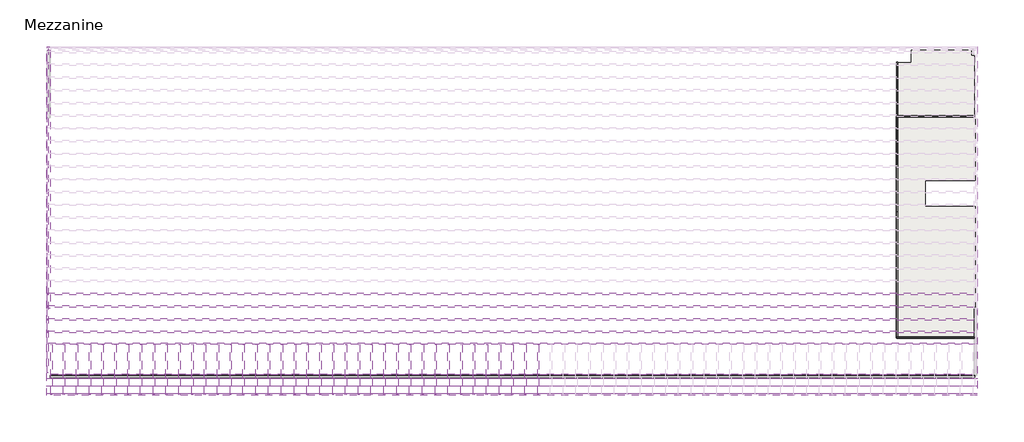
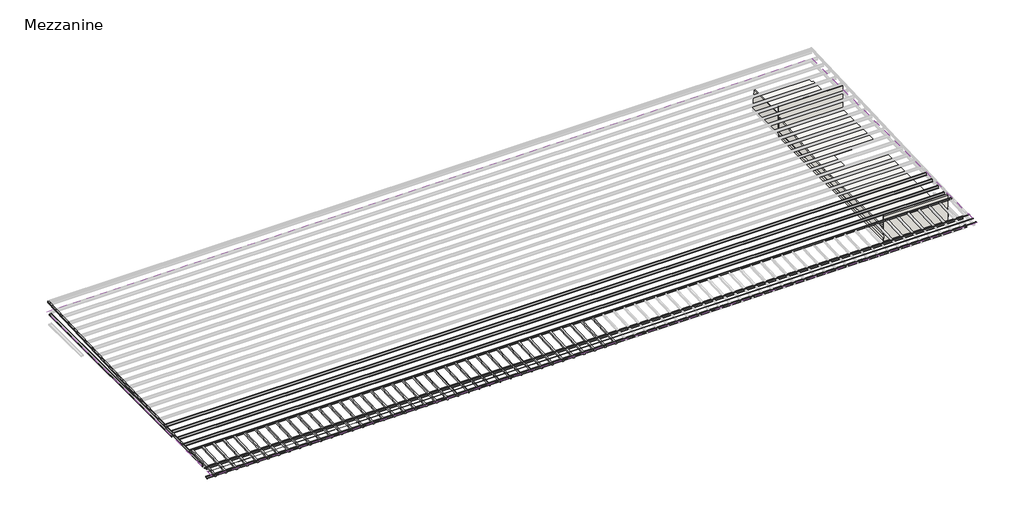
# One storey, part 1 of 2: 51 beams, 4 walls, 2 slabs, 1 roof.
"""IFC4 building model written with IfcOpenShell, lengths in millimetres."""

import ifcopenshell
import ifcopenshell.guid

model = None  # the IFC model being written
_history = None  # IfcOwnerHistory: only IFC2X3 demands one
_inside = {}  # id of a spatial element -> (the spatial element, [elements in it])
_under = {}  # id of a project, library or spatial element -> (it, [spatial elements below it])
_declared = {}  # id of a project -> (the project, [libraries it declares])
_typed = {}  # id of a type object -> (the type object, [elements of that type])
_made_of = {}  # id of a material, layer set ... -> (it, [elements and type objects made of it])


def new_model(schema):
    """Start an empty IFC model of exactly this schema.

    Asked for "IFC4X3", IfcOpenShell would pick the latest addendum, in which some entities
    have other attributes; the version numbers below select the first issue.
    IFC2X3 requires an IfcOwnerHistory on every rooted entity: one is made here for all.
    """
    global model, _history
    if schema == "IFC4X3":
        model = ifcopenshell.file(schema_version=(4, 3, 0, 0))
    else:
        model = ifcopenshell.file(schema=schema)
    _inside.clear()
    _under.clear()
    _declared.clear()
    _typed.clear()
    _made_of.clear()
    _history = None
    if model.schema == "IFC2X3":
        org = make("IfcOrganization", Name="unknown")
        user = make(
            "IfcPersonAndOrganization",
            ThePerson=make("IfcPerson", FamilyName="unknown"),
            TheOrganization=org,
        )
        app = make(
            "IfcApplication",
            ApplicationDeveloper=org,
            Version="unknown",
            ApplicationFullName="unknown",
            ApplicationIdentifier="unknown",
        )
        _history = make(
            "IfcOwnerHistory",
            OwningUser=user,
            OwningApplication=app,
            ChangeAction="ADDED",
            CreationDate=0,
        )
    return model


def make(cls, **values):
    """One entity of the class cls with the attributes given. An attribute that is None is left unset."""
    return model.create_entity(
        cls, **{name: value for name, value in values.items() if value is not None}
    )


def rooted(cls, **values):
    """An entity with a GlobalId (a new one), such as an element, a storey or a relation."""
    return make(cls, GlobalId=ifcopenshell.guid.new(), OwnerHistory=_history, **values)


def si_unit(unit_type, name, prefix=None):
    """IfcSIUnit, for example si_unit("LENGTHUNIT", "METRE", prefix="MILLI")."""
    return make("IfcSIUnit", UnitType=unit_type, Prefix=prefix, Name=name)


def assignment(units):
    """IfcUnitAssignment: the units of a project."""
    return None if units is None else make("IfcUnitAssignment", Units=units)


def point(xyz):
    """IfcCartesianPoint."""
    return None if xyz is None else make("IfcCartesianPoint", Coordinates=xyz)


def direction(xyz):
    """IfcDirection."""
    return None if xyz is None else make("IfcDirection", DirectionRatios=xyz)


def frame(location, z_axis=None, x_axis=None):
    """IfcAxis2Placement3D, a coordinate frame: its origin and axes. An axis left out is left unset."""
    return make(
        "IfcAxis2Placement3D",
        Location=point(location),
        Axis=direction(z_axis),
        RefDirection=direction(x_axis),
    )


def frame_2d(location, x_axis=None):
    """IfcAxis2Placement2D, a coordinate frame in the plane: its origin and x axis."""
    return make(
        "IfcAxis2Placement2D", Location=point(location), RefDirection=direction(x_axis)
    )


def origin():
    """The frame at (0, 0, 0) with its axes left unset."""
    return frame((0.0, 0.0, 0.0))


def place(relative_to, where):
    """IfcLocalPlacement: puts the frame where relative to a parent placement (None: the world)."""
    return make(
        "IfcLocalPlacement", PlacementRelTo=relative_to, RelativePlacement=where
    )


def context(
    kind, dimensions, precision=None, world=None, true_north=None, identifier=None
):
    """IfcGeometricRepresentationContext, for example the 3D "Model" context."""
    return make(
        "IfcGeometricRepresentationContext",
        ContextIdentifier=identifier,
        ContextType=kind,
        CoordinateSpaceDimension=dimensions,
        Precision=precision,
        WorldCoordinateSystem=world,
        TrueNorth=true_north,
    )


def project(units=None, contexts=None):
    """IfcProject with its units and contexts."""
    return rooted(
        "IfcProject",
        Name="project",
        RepresentationContexts=contexts,
        UnitsInContext=assignment(units),
    )


def spatial(cls, under=None, at=None, **own):
    """A site, building, storey or space (cls), placed at a placement, below another one or the project."""
    s = rooted(cls, ObjectPlacement=at, **own)
    if under is not None:
        _under.setdefault(under.id(), (under, []))[1].append(s)
    return s


def polyline(points):
    """IfcPolyline through the points."""
    return make("IfcPolyline", Points=[point(p) for p in points])


def circle_curve(where, radius):
    """IfcCircle in the frame where."""
    return make("IfcCircle", Position=where, Radius=radius)


def trimmed(basis, trim1, trim2, sense, master):
    """IfcTrimmedCurve: the piece of a basis curve between two trims."""
    return make(
        "IfcTrimmedCurve",
        BasisCurve=basis,
        Trim1=trim1,
        Trim2=trim2,
        SenseAgreement=sense,
        MasterRepresentation=master,
    )


def segment(curve, same_sense, transition):
    """IfcCompositeCurveSegment."""
    return make(
        "IfcCompositeCurveSegment",
        Transition=transition,
        SameSense=same_sense,
        ParentCurve=curve,
    )


def composite_curve(segments, self_intersect=None):
    """IfcCompositeCurve: segments joined end to end."""
    return make("IfcCompositeCurve", Segments=segments, SelfIntersect=self_intersect)


def outline(outer, holes=None, kind="AREA"):
    """IfcArbitraryClosedProfileDef: a profile drawn as a closed curve; with holes, ...WithVoids."""
    if holes is None:
        return make("IfcArbitraryClosedProfileDef", ProfileType=kind, OuterCurve=outer)
    return make(
        "IfcArbitraryProfileDefWithVoids",
        ProfileType=kind,
        OuterCurve=outer,
        InnerCurves=holes,
    )


def extrude(swept, where, along, depth):
    """IfcExtrudedAreaSolid: the profile swept, set in the frame where, extruded along a direction by depth."""
    return make(
        "IfcExtrudedAreaSolid",
        SweptArea=swept,
        Position=where,
        ExtrudedDirection=direction(along),
        Depth=depth,
    )


def faces_of(points, faces, orient=None, outer=None):
    """IfcFace entities. A face is a list of loops; a loop is a list of indices into points, from 0.

    orient and outer hold one flag for each loop. By default every Orientation is true, the
    first loop of a face is its IfcFaceOuterBound and the others are IfcFaceBound.
    """
    made = []
    for i, loops in enumerate(faces):
        bounds = []
        for j, loop in enumerate(loops):
            is_outer = j == 0 if outer is None else outer[i][j]
            bounds.append(
                make(
                    "IfcFaceOuterBound" if is_outer else "IfcFaceBound",
                    Bound=make("IfcPolyLoop", Polygon=[points[k] for k in loop]),
                    Orientation=True if orient is None else orient[i][j],
                )
            )
        made.append(make("IfcFace", Bounds=bounds))
    return made


def faceted_brep(points, faces, orient=None, outer=None, voids=None):
    """IfcFacetedBrep: a solid bounded by flat faces; with voids (closed shells), ...WithVoids."""
    shared = [point(p) for p in points]
    hull = make("IfcClosedShell", CfsFaces=faces_of(shared, faces, orient, outer))
    if voids is None:
        return make("IfcFacetedBrep", Outer=hull)
    return make(
        "IfcFacetedBrepWithVoids",
        Outer=hull,
        Voids=[
            make(cls, CfsFaces=faces_of(shared, fs, o, b)) for cls, fs, o, b in voids
        ],
    )


def shape(context_of_items, identifier, shape_type, items):
    """IfcShapeRepresentation: the items that make up one representation, for example the "Body"."""
    return make(
        "IfcShapeRepresentation",
        ContextOfItems=context_of_items,
        RepresentationIdentifier=identifier,
        RepresentationType=shape_type,
        Items=items,
    )


def source(mapping_origin, context_of_items, identifier, shape_type, items):
    """IfcRepresentationMap: a shape defined once, which mapped items show again and again."""
    return make(
        "IfcRepresentationMap",
        MappingOrigin=mapping_origin,
        MappedRepresentation=shape(context_of_items, identifier, shape_type, items),
    )


def transform(
    local_origin,
    x_axis=None,
    y_axis=None,
    z_axis=None,
    scale=None,
    scale2=None,
    scale3=None,
    uniform=True,
):
    """IfcCartesianTransformationOperator3D, or its non-uniform kind. x_axis, y_axis, z_axis: its Axis1, 2, 3."""
    if uniform:
        return make(
            "IfcCartesianTransformationOperator3D",
            Axis1=direction(x_axis),
            Axis2=direction(y_axis),
            LocalOrigin=point(local_origin),
            Scale=scale,
            Axis3=direction(z_axis),
        )
    return make(
        "IfcCartesianTransformationOperator3DnonUniform",
        Axis1=direction(x_axis),
        Axis2=direction(y_axis),
        LocalOrigin=point(local_origin),
        Scale=scale,
        Axis3=direction(z_axis),
        Scale2=scale2,
        Scale3=scale3,
    )


def mapped(mapping_source, mapping_target):
    """IfcMappedItem: shows the shape of a source again, moved by a transform."""
    return make(
        "IfcMappedItem", MappingSource=mapping_source, MappingTarget=mapping_target
    )


def made_of(thing, what):
    """Note that an element or type object is made of a material, layer set ...; save() writes the relation."""
    if what is not None:
        _made_of.setdefault(what.id(), (what, []))[1].append(thing)
    return thing


def element(
    cls,
    number,
    at=None,
    inside=None,
    cuts=None,
    type_object=None,
    material=None,
    context=None,
    identifier="Body",
    shape_type=None,
    held_by="IfcProductDefinitionShape",
    body=None,
    shapes=None,
    **own,
):
    """One element of the class cls, such as IfcWall. Its Tag is "e" and its number.

    at: its placement. inside: the storey or other place that contains it. cuts: it is an
    opening in that element (IfcRelVoidsElement). A single representation is given by context,
    identifier, shape_type and body (its items); several are given by shapes. held_by: the class
    of the entity that holds the representations. save() writes the other relations.
    """
    e = rooted(cls, Tag="e%d" % number, ObjectPlacement=at, **own)
    if body is not None:
        shapes = [shape(context, identifier, shape_type, body)]
    if shapes is not None:
        e.Representation = make(held_by, Representations=shapes)
    if inside is not None:
        _inside.setdefault(inside.id(), (inside, []))[1].append(e)
    if cuts is not None:
        rooted(
            "IfcRelVoidsElement", RelatingBuildingElement=cuts, RelatedOpeningElement=e
        )
    if type_object is not None:
        _typed.setdefault(type_object.id(), (type_object, []))[1].append(e)
    return made_of(e, material)


def aggregate(whole, parts):
    """IfcRelAggregates: a whole, such as a stair, and the parts it consists of."""
    return rooted("IfcRelAggregates", RelatingObject=whole, RelatedObjects=parts)


def save(model, path):
    """Write the relations noted so far, then the file.

    IfcRelAggregates (storeys below a building ...), IfcRelContainedInSpatialStructure (elements
    in a storey), IfcRelDefinesByType, IfcRelAssociatesMaterial and IfcRelDeclares: one each for
    every whole, place, type object, material and project.
    """
    for whole, parts in _under.values():
        aggregate(whole, parts)
    for where, things in _inside.values():
        rooted(
            "IfcRelContainedInSpatialStructure",
            RelatedElements=things,
            RelatingStructure=where,
        )
    for kind, things in _typed.values():
        rooted("IfcRelDefinesByType", RelatedObjects=things, RelatingType=kind)
    for what, things in _made_of.values():
        rooted("IfcRelAssociatesMaterial", RelatedObjects=things, RelatingMaterial=what)
    for by, libraries in _declared.values():
        rooted("IfcRelDeclares", RelatingContext=by, RelatedDefinitions=libraries)
    model.write(path)


def dimension_lumber_5_5_x_7_5_glulam_5a1f9f63(model_context):
    return source(origin(), model_context, "Body", "SweptSolid", [
        extrude(outline(polyline([(2439.95575, 69.85), (2439.95575, -69.85), (-2389.02875, -69.85), (-2389.02875, 69.85), (2439.95575, 69.85)])), frame((0.0, 0.0, -95.25), z_axis=(0.0, 0.0, 1.0), x_axis=(1.0, 0.0, 0.0)), (0.0, 0.0, 1.0), 190.5),
    ])


def beam_b6572ddd(model_context):
    return source(origin(), model_context, "Body", "SweptSolid", [
        extrude(outline(composite_curve([segment(polyline([(87.5109375, 101.6), (99.7560415, 87.0068534), (97.6278742, 85.221109), (86.2154765, 98.821875), (3.3005807, 98.821875)]), True, "CONTINUOUS"), segment(trimmed(circle_curve(frame_2d((3.3741066, 96.8381931)), 1.9850441), [point((3.3005807, 98.821875))], [point((1.3890625, 96.8381931))], True, "CARTESIAN"), True, "CONTINUOUS"), segment(polyline([(1.3890625, 96.8381931), (1.3890625, -96.8389339)]), True, "CONTINUOUS"), segment(trimmed(circle_curve(frame_2d((3.3748024, -96.8389339)), 1.9857399), [point((1.3890625, -96.8389339))], [point((3.2694106, -98.821875))], True, "CARTESIAN"), True, "CONTINUOUS"), segment(polyline([(3.2694106, -98.821875), (86.2154765, -98.821875), (97.6510975, -85.1934327), (99.7792647, -86.979177), (87.5109375, -101.6), (3.3734375, -101.6)]), True, "CONTINUOUS"), segment(trimmed(circle_curve(frame_2d((3.3734375, -96.8375)), 4.7625), [point((3.3734375, -101.6))], [point((-1.3890625, -96.8375))], False, "CARTESIAN"), True, "CONTINUOUS"), segment(polyline([(-1.3890625, -96.8375), (-1.3890625, 96.8375)]), True, "CONTINUOUS"), segment(trimmed(circle_curve(frame_2d((3.3734375, 96.8375)), 4.7625), [point((-1.3890625, 96.8375))], [point((3.3734375, 101.6))], False, "CARTESIAN"), True, "CONTINUOUS"), segment(polyline([(3.3734375, 101.6), (87.5109375, 101.6)]), True, "CONTINUOUS")], self_intersect=False)), frame((-15570.2, 0.0, 0.0), z_axis=(1.0, 0.0, 0.0), x_axis=(0.0, 1.0, 0.0)), (0.0, 0.0, 1.0), 31140.4),
    ])


def beam_b1d2936f(model_context):
    return source(origin(), model_context, "Body", "SweptSolid", [
        extrude(outline(composite_curve([segment(polyline([(-77.9859375, 127.0), (-3.3734375, 127.0)]), True, "CONTINUOUS"), segment(trimmed(circle_curve(frame_2d((-3.3734375, 122.2375)), 4.7625), [point((-3.3734375, 127.0))], [point((1.3890625, 122.2375))], False, "CARTESIAN"), True, "CONTINUOUS"), segment(polyline([(1.3890625, 122.2375), (1.3890625, -122.2389339)]), True, "CONTINUOUS"), segment(trimmed(circle_curve(frame_2d((3.3748024, -122.2389339)), 1.9857399), [point((1.3890625, -122.2389339))], [point((3.2694106, -124.221875))], True, "CARTESIAN"), True, "CONTINUOUS"), segment(polyline([(3.2694106, -124.221875), (83.0404765, -124.221875), (94.4528742, -110.621109), (96.5810415, -112.4068534), (84.3359375, -127.0), (-1.3890625, -127.0), (-1.3890625, 122.2381931)]), True, "CONTINUOUS"), segment(trimmed(circle_curve(frame_2d((-3.3741066, 122.2381931)), 1.9850441), [point((-1.3890625, 122.2381931))], [point((-3.3005807, 124.221875))], True, "CARTESIAN"), True, "CONTINUOUS"), segment(polyline([(-3.3005807, 124.221875), (-76.6904765, 124.221875), (-88.1028742, 110.621109), (-90.2310415, 112.4068534), (-77.9859375, 127.0)]), True, "CONTINUOUS")], self_intersect=False)), frame((-44221.4, 0.0, 0.0), z_axis=(1.0, 0.0, 0.0), x_axis=(0.0, 1.0, 0.0)), (0.0, 0.0, 1.0), 88442.8),
    ])


def beam_302408e8(model_context):
    return source(origin(), model_context, "Body", "SweptSolid", [
        extrude(outline(composite_curve([segment(polyline([(77.9859375, 127.0), (90.2310415, 112.4068534), (88.1028742, 110.621109), (76.6904765, 124.221875), (3.3005807, 124.221875)]), True, "CONTINUOUS"), segment(trimmed(circle_curve(frame_2d((3.3741066, 122.2381931)), 1.9850441), [point((3.3005807, 124.221875))], [point((1.3890625, 122.2381931))], True, "CARTESIAN"), True, "CONTINUOUS"), segment(polyline([(1.3890625, 122.2381931), (1.3890625, -127.0), (-84.3359375, -127.0), (-96.5810415, -112.4068534), (-94.4528742, -110.621109), (-83.0404765, -124.221875), (-3.2694106, -124.221875)]), True, "CONTINUOUS"), segment(trimmed(circle_curve(frame_2d((-3.3748024, -122.2389339)), 1.9857399), [point((-3.2694106, -124.221875))], [point((-1.3890625, -122.2389339))], True, "CARTESIAN"), True, "CONTINUOUS"), segment(polyline([(-1.3890625, -122.2389339), (-1.3890625, 122.2375)]), True, "CONTINUOUS"), segment(trimmed(circle_curve(frame_2d((3.3734375, 122.2375)), 4.7625), [point((-1.3890625, 122.2375))], [point((3.3734375, 127.0))], False, "CARTESIAN"), True, "CONTINUOUS"), segment(polyline([(3.3734375, 127.0), (77.9859375, 127.0)]), True, "CONTINUOUS")], self_intersect=False)), frame((-12455.525, 0.0, 0.0), z_axis=(1.0, 0.0, 0.0), x_axis=(0.0, 1.0, 0.0)), (0.0, 0.0, 1.0), 24739.6),
    ])


def beam_bf61a610(model_context):
    return source(origin(), model_context, "Body", "SweptSolid", [
        extrude(outline(composite_curve([segment(polyline([(77.9859375, 127.0), (90.2310415, 112.4068534), (88.1028742, 110.621109), (76.6904765, 124.221875), (3.3005807, 124.221875)]), True, "CONTINUOUS"), segment(trimmed(circle_curve(frame_2d((3.3741066, 122.2381931)), 1.9850441), [point((3.3005807, 124.221875))], [point((1.3890625, 122.2381931))], True, "CARTESIAN"), True, "CONTINUOUS"), segment(polyline([(1.3890625, 122.2381931), (1.3890625, -127.0), (-84.3359375, -127.0), (-96.5810415, -112.4068534), (-94.4528742, -110.621109), (-83.0404765, -124.221875), (-3.2694106, -124.221875)]), True, "CONTINUOUS"), segment(trimmed(circle_curve(frame_2d((-3.3748024, -122.2389339)), 1.9857399), [point((-3.2694106, -124.221875))], [point((-1.3890625, -122.2389339))], True, "CARTESIAN"), True, "CONTINUOUS"), segment(polyline([(-1.3890625, -122.2389339), (-1.3890625, 122.2375)]), True, "CONTINUOUS"), segment(trimmed(circle_curve(frame_2d((3.3734375, 122.2375)), 4.7625), [point((-1.3890625, 122.2375))], [point((3.3734375, 127.0))], False, "CARTESIAN"), True, "CONTINUOUS"), segment(polyline([(3.3734375, 127.0), (77.9859375, 127.0)]), True, "CONTINUOUS")], self_intersect=False)), frame((-44283.1884767, 0.0, 0.0), z_axis=(1.0, 0.0, 0.0), x_axis=(0.0, 1.0, 0.0)), (0.0, 0.0, 1.0), 88566.3769533),
    ])


def hss_hollow_structural_section_hss1_1_2x1_1_2x1_8_obsolete_11a1fb5f(model_context):
    return source(origin(), model_context, "Body", "SweptSolid", [
        extrude(outline(composite_curve([segment(polyline([(19.05, 13.1572), (19.05, -13.1572)]), True, "CONTINUOUS"), segment(trimmed(circle_curve(frame_2d((13.1572, -13.1572)), 5.8928), [point((19.05, -13.1572))], [point((13.1572, -19.05))], False, "CARTESIAN"), True, "CONTINUOUS"), segment(polyline([(13.1572, -19.05), (-13.1572, -19.05)]), True, "CONTINUOUS"), segment(trimmed(circle_curve(frame_2d((-13.1572, -13.1572)), 5.8928), [point((-13.1572, -19.05))], [point((-19.05, -13.1572))], False, "CARTESIAN"), True, "CONTINUOUS"), segment(polyline([(-19.05, -13.1572), (-19.05, 13.1572)]), True, "CONTINUOUS"), segment(trimmed(circle_curve(frame_2d((-13.1572, 13.1572)), 5.8928), [point((-19.05, 13.1572))], [point((-13.1572, 19.05))], False, "CARTESIAN"), True, "CONTINUOUS"), segment(polyline([(-13.1572, 19.05), (13.1572, 19.05)]), True, "CONTINUOUS"), segment(trimmed(circle_curve(frame_2d((13.1572, 13.1572)), 5.8928), [point((13.1572, 19.05))], [point((19.05, 13.1572))], False, "CARTESIAN"), True, "CONTINUOUS")], self_intersect=False), holes=[composite_curve([segment(trimmed(circle_curve(frame_2d((-13.1572, 13.1572)), 2.9464), [point((-13.1572, 16.1036))], [point((-16.1036, 13.1572))], True, "CARTESIAN"), True, "CONTINUOUS"), segment(polyline([(-16.1036, 13.1572), (-16.1036, -13.1572)]), True, "CONTINUOUS"), segment(trimmed(circle_curve(frame_2d((-13.1572, -13.1572)), 2.9464), [point((-16.1036, -13.1572))], [point((-13.1572, -16.1036))], True, "CARTESIAN"), True, "CONTINUOUS"), segment(polyline([(-13.1572, -16.1036), (13.1572, -16.1036)]), True, "CONTINUOUS"), segment(trimmed(circle_curve(frame_2d((13.1572, -13.1572)), 2.9464), [point((13.1572, -16.1036))], [point((16.1036, -13.1572))], True, "CARTESIAN"), True, "CONTINUOUS"), segment(polyline([(16.1036, -13.1572), (16.1036, 13.1572)]), True, "CONTINUOUS"), segment(trimmed(circle_curve(frame_2d((13.1572, 13.1572)), 2.9464), [point((16.1036, 13.1572))], [point((13.1572, 16.1036))], True, "CARTESIAN"), True, "CONTINUOUS"), segment(polyline([(13.1572, 16.1036), (-13.1572, 16.1036)]), True, "CONTINUOUS")], self_intersect=False)]), frame((-44523.0377, 0.0, 0.0), z_axis=(1.0, 0.0, 0.0), x_axis=(0.0, 1.0, 0.0)), (0.0, 0.0, 1.0), 89046.0754),
    ])


def w_wide_flange_w12x19_f5d0d782(model_context):
    return source(origin(), model_context, "Body", "SweptSolid", [
        extrude(outline(composite_curve([segment(polyline([(50.927, -146.05), (50.927, -154.94), (-50.927, -154.94), (-50.927, -146.05), (-16.3195, -146.05)]), True, "CONTINUOUS"), segment(trimmed(circle_curve(frame_2d((-16.3195, -132.715)), 13.335), [point((-16.3195, -146.05))], [point((-2.9845, -132.715))], True, "CARTESIAN"), True, "CONTINUOUS"), segment(polyline([(-2.9845, -132.715), (-2.9845, 132.715)]), True, "CONTINUOUS"), segment(trimmed(circle_curve(frame_2d((-16.3195, 132.715)), 13.335), [point((-2.9845, 132.715))], [point((-16.3195, 146.05))], True, "CARTESIAN"), True, "CONTINUOUS"), segment(polyline([(-16.3195, 146.05), (-50.927, 146.05), (-50.927, 154.94), (50.927, 154.94), (50.927, 146.05), (16.3195, 146.05)]), True, "CONTINUOUS"), segment(trimmed(circle_curve(frame_2d((16.3195, 132.715)), 13.335), [point((16.3195, 146.05))], [point((2.9845, 132.715))], True, "CARTESIAN"), True, "CONTINUOUS"), segment(polyline([(2.9845, 132.715), (2.9845, -132.715)]), True, "CONTINUOUS"), segment(trimmed(circle_curve(frame_2d((16.3195, -132.715)), 13.335), [point((2.9845, -132.715))], [point((16.3195, -146.05))], True, "CARTESIAN"), True, "CONTINUOUS"), segment(polyline([(16.3195, -146.05), (50.927, -146.05)]), True, "CONTINUOUS")], self_intersect=False)), frame((-44073.7625, 0.0, 0.0), z_axis=(1.0, 0.0, 0.0), x_axis=(0.0, 1.0, 0.0)), (0.0, 0.0, 1.0), 88074.5),
    ])


def w_wide_flange_w8x15_6c148e4e(model_context):
    return source(origin(), model_context, "Body", "SweptSolid", [
        extrude(outline(composite_curve([segment(polyline([(50.927, -94.996), (50.927, -102.997), (-50.927, -102.997), (-50.927, -94.996), (-15.748, -94.996)]), True, "CONTINUOUS"), segment(trimmed(circle_curve(frame_2d((-15.748, -82.3595)), 12.6365), [point((-15.748, -94.996))], [point((-3.1115, -82.3595))], True, "CARTESIAN"), True, "CONTINUOUS"), segment(polyline([(-3.1115, -82.3595), (-3.1115, 82.3595)]), True, "CONTINUOUS"), segment(trimmed(circle_curve(frame_2d((-15.748, 82.3595)), 12.6365), [point((-3.1115, 82.3595))], [point((-15.748, 94.996))], True, "CARTESIAN"), True, "CONTINUOUS"), segment(polyline([(-15.748, 94.996), (-50.927, 94.996), (-50.927, 102.997), (50.927, 102.997), (50.927, 94.996), (15.748, 94.996)]), True, "CONTINUOUS"), segment(trimmed(circle_curve(frame_2d((15.748, 82.3595)), 12.6365), [point((15.748, 94.996))], [point((3.1115, 82.3595))], True, "CARTESIAN"), True, "CONTINUOUS"), segment(polyline([(3.1115, 82.3595), (3.1115, -82.3595)]), True, "CONTINUOUS"), segment(trimmed(circle_curve(frame_2d((15.748, -82.3595)), 12.6365), [point((3.1115, -82.3595))], [point((15.748, -94.996))], True, "CARTESIAN"), True, "CONTINUOUS"), segment(polyline([(15.748, -94.996), (50.927, -94.996)]), True, "CONTINUOUS")], self_intersect=False)), frame((-44289.8957353, 0.0, 0.0), z_axis=(1.0, 0.0, 0.0), x_axis=(0.0, 1.0, 0.0)), (0.0, 0.0, 1.0), 88692.2707353),
    ])


model = new_model("IFC4")

# Units and contexts
model_context = context("Model", 3, world=origin())
ifc_project = project(units=[si_unit("LENGTHUNIT", "METRE", prefix="MILLI")], contexts=[model_context])

# Site, building, storey
site = spatial("IfcSite", under=ifc_project)
building = spatial("IfcBuilding", under=site)
storey = spatial("IfcBuildingStorey", under=building, Name="Mezzanine", Elevation=6553.2)

# Beams
placement = place(None, origin())
dimension_lumber_5_5_x_7_5_glulam_shape = dimension_lumber_5_5_x_7_5_glulam_5a1f9f63(model_context)
element("IfcBeam", 1, ObjectType="Dimension Lumber : 5.5 x 7.5 Glulam", at=placement, inside=storey, context=model_context, shape_type="MappedRepresentation", body=[
    mapped(dimension_lumber_5_5_x_7_5_glulam_shape, transform((625599.2117243, -567351.2774558, 8705.0370798), x_axis=(0.0, -0.999133073092352, -0.04163054471217889), y_axis=(1.0, 0.0, 0.0), z_axis=(0.0, -0.0416305447121789, 0.9991330730923521))),
])
element("IfcBeam", 2, ObjectType="Dimension Lumber : 5.5 x 7.5 Glulam", at=placement, inside=storey, context=model_context, shape_type="MappedRepresentation", body=[
    mapped(dimension_lumber_5_5_x_7_5_glulam_shape, transform((624373.6617243, -567351.2774558, 8705.0370798), x_axis=(0.0, -0.999133073092352, -0.04163054471217889), y_axis=(1.0, 0.0, 0.0), z_axis=(0.0, -0.04163054471217882, 0.9991330730923521))),
])
element("IfcBeam", 3, ObjectType="Dimension Lumber : 5.5 x 7.5 Glulam", at=placement, inside=storey, context=model_context, shape_type="MappedRepresentation", body=[
    mapped(dimension_lumber_5_5_x_7_5_glulam_shape, transform((623148.1117243, -567351.2774558, 8705.0370798), x_axis=(0.0, -0.999133073092352, -0.04163054471217911), y_axis=(1.0, 0.0, 0.0), z_axis=(0.0, -0.04163054471217904, 0.9991330730923521))),
])
element("IfcBeam", 4, ObjectType="Dimension Lumber : 5.5 x 7.5 Glulam", at=placement, inside=storey, context=model_context, shape_type="MappedRepresentation", body=[
    mapped(dimension_lumber_5_5_x_7_5_glulam_shape, transform((621922.5617243, -567351.2774558, 8705.0370798), x_axis=(0.0, -0.999133073092352, -0.04163054471217889), y_axis=(1.0, 0.0, 0.0), z_axis=(0.0, -0.0416305447121789, 0.9991330730923521))),
])
element("IfcBeam", 5, ObjectType="Dimension Lumber : 5.5 x 7.5 Glulam", at=placement, inside=storey, context=model_context, shape_type="MappedRepresentation", body=[
    mapped(dimension_lumber_5_5_x_7_5_glulam_shape, transform((620697.0117243, -567351.2774558, 8705.0370798), x_axis=(0.0, -0.999133073092352, -0.04163054471217889), y_axis=(1.0, 0.0, 0.0), z_axis=(0.0, -0.04163054471217882, 0.9991330730923521))),
])
element("IfcBeam", 6, ObjectType="Dimension Lumber : 5.5 x 7.5 Glulam", at=placement, inside=storey, context=model_context, shape_type="MappedRepresentation", body=[
    mapped(dimension_lumber_5_5_x_7_5_glulam_shape, transform((619471.4617243, -567351.2774558, 8705.0370798), x_axis=(0.0, -0.999133073092352, -0.04163054471217911), y_axis=(1.0, 0.0, 0.0), z_axis=(0.0, -0.04163054471217912, 0.9991330730923521))),
])
element("IfcBeam", 7, ObjectType="Dimension Lumber : 5.5 x 7.5 Glulam", at=placement, inside=storey, context=model_context, shape_type="MappedRepresentation", body=[
    mapped(dimension_lumber_5_5_x_7_5_glulam_shape, transform((618245.9117243, -567351.2774558, 8705.0370798), x_axis=(0.0, -0.999133073092352, -0.04163054471217889), y_axis=(1.0, 0.0, 0.0), z_axis=(0.0, -0.0416305447121789, 0.9991330730923521))),
])
element("IfcBeam", 8, ObjectType="Dimension Lumber : 5.5 x 7.5 Glulam", at=placement, inside=storey, context=model_context, shape_type="MappedRepresentation", body=[
    mapped(dimension_lumber_5_5_x_7_5_glulam_shape, transform((617020.3617243, -567351.2774558, 8705.0370798), x_axis=(0.0, -0.999133073092352, -0.04163054471217889), y_axis=(1.0, 0.0, 0.0), z_axis=(0.0, -0.04163054471217882, 0.9991330730923521))),
])
element("IfcBeam", 9, ObjectType="Dimension Lumber : 5.5 x 7.5 Glulam", at=placement, inside=storey, context=model_context, shape_type="MappedRepresentation", body=[
    mapped(dimension_lumber_5_5_x_7_5_glulam_shape, transform((615794.8117243, -567351.2774558, 8705.0370798), x_axis=(0.0, -0.999133073092352, -0.04163054471217911), y_axis=(1.0, 0.0, 0.0), z_axis=(0.0, -0.04163054471217912, 0.9991330730923521))),
])
element("IfcBeam", 10, ObjectType="Dimension Lumber : 5.5 x 7.5 Glulam", at=placement, inside=storey, context=model_context, shape_type="MappedRepresentation", body=[
    mapped(dimension_lumber_5_5_x_7_5_glulam_shape, transform((614569.2617243, -567351.2774558, 8705.0370798), x_axis=(0.0, -0.999133073092352, -0.04163054471217889), y_axis=(1.0, 0.0, 0.0), z_axis=(0.0, -0.0416305447121789, 0.9991330730923521))),
])
element("IfcBeam", 11, ObjectType="Dimension Lumber : 5.5 x 7.5 Glulam", at=placement, inside=storey, context=model_context, shape_type="MappedRepresentation", body=[
    mapped(dimension_lumber_5_5_x_7_5_glulam_shape, transform((613343.7117243, -567351.2774558, 8705.0370798), x_axis=(0.0, -0.999133073092352, -0.04163054471217889), y_axis=(1.0, 0.0, 0.0), z_axis=(0.0, -0.04163054471217882, 0.9991330730923521))),
])
element("IfcBeam", 12, ObjectType="Dimension Lumber : 5.5 x 7.5 Glulam", at=placement, inside=storey, context=model_context, shape_type="MappedRepresentation", body=[
    mapped(dimension_lumber_5_5_x_7_5_glulam_shape, transform((612118.1617243, -567351.2774558, 8705.0370798), x_axis=(0.0, -0.999133073092352, -0.04163054471217889), y_axis=(1.0, 0.0, 0.0), z_axis=(0.0, -0.0416305447121789, 0.9991330730923521))),
])
element("IfcBeam", 13, ObjectType="Dimension Lumber : 5.5 x 7.5 Glulam", at=placement, inside=storey, context=model_context, shape_type="MappedRepresentation", body=[
    mapped(dimension_lumber_5_5_x_7_5_glulam_shape, transform((610892.6117243, -567351.2774558, 8705.0370798), x_axis=(0.0, -0.999133073092352, -0.04163054471217889), y_axis=(1.0, 0.0, 0.0), z_axis=(0.0, -0.0416305447121789, 0.9991330730923521))),
])
element("IfcBeam", 14, ObjectType="Dimension Lumber : 5.5 x 7.5 Glulam", at=placement, inside=storey, context=model_context, shape_type="MappedRepresentation", body=[
    mapped(dimension_lumber_5_5_x_7_5_glulam_shape, transform((609667.0617243, -567351.2774558, 8705.0370798), x_axis=(0.0, -0.999133073092352, -0.04163054471217889), y_axis=(1.0, 0.0, 0.0), z_axis=(0.0, -0.041630544712178974, 0.9991330730923521))),
])
element("IfcBeam", 15, ObjectType="Dimension Lumber : 5.5 x 7.5 Glulam", at=placement, inside=storey, context=model_context, shape_type="MappedRepresentation", body=[
    mapped(dimension_lumber_5_5_x_7_5_glulam_shape, transform((608441.5117243, -567351.2774558, 8705.0370798), x_axis=(0.0, -0.999133073092352, -0.04163054471217889), y_axis=(1.0, 0.0, 0.0), z_axis=(0.0, -0.0416305447121789, 0.9991330730923521))),
])
element("IfcBeam", 16, ObjectType="Dimension Lumber : 5.5 x 7.5 Glulam", at=placement, inside=storey, context=model_context, shape_type="MappedRepresentation", body=[
    mapped(dimension_lumber_5_5_x_7_5_glulam_shape, transform((607215.9617243, -567351.2774558, 8705.0370798), x_axis=(0.0, -0.999133073092352, -0.04163054471217889), y_axis=(1.0, 0.0, 0.0), z_axis=(0.0, -0.0416305447121789, 0.9991330730923521))),
])
element("IfcBeam", 17, ObjectType="Dimension Lumber : 5.5 x 7.5 Glulam", at=placement, inside=storey, context=model_context, shape_type="MappedRepresentation", body=[
    mapped(dimension_lumber_5_5_x_7_5_glulam_shape, transform((605990.4117243, -567351.2774558, 8705.0370798), x_axis=(0.0, -0.999133073092352, -0.04163054471217911), y_axis=(0.9999999999999999, 0.0, 0.0), z_axis=(0.0, -0.04163054471217919, 0.999133073092352))),
])
element("IfcBeam", 18, ObjectType="Dimension Lumber : 5.5 x 7.5 Glulam", at=placement, inside=storey, context=model_context, shape_type="MappedRepresentation", body=[
    mapped(dimension_lumber_5_5_x_7_5_glulam_shape, transform((604764.8617243, -567351.2774558, 8705.0370798), x_axis=(0.0, -0.999133073092352, -0.04163054471217889), y_axis=(1.0, 0.0, 0.0), z_axis=(0.0, -0.0416305447121789, 0.9991330730923521))),
])
element("IfcBeam", 19, ObjectType="Dimension Lumber : 5.5 x 7.5 Glulam", at=placement, inside=storey, context=model_context, shape_type="MappedRepresentation", body=[
    mapped(dimension_lumber_5_5_x_7_5_glulam_shape, transform((603539.3117243, -567351.2774558, 8705.0370798), x_axis=(0.0, -0.999133073092352, -0.04163054471217889), y_axis=(1.0, 0.0, 0.0), z_axis=(0.0, -0.041630544712178974, 0.9991330730923521))),
])
element("IfcBeam", 20, ObjectType="Dimension Lumber : 5.5 x 7.5 Glulam", at=placement, inside=storey, context=model_context, shape_type="MappedRepresentation", body=[
    mapped(dimension_lumber_5_5_x_7_5_glulam_shape, transform((602313.7617243, -567351.2774558, 8705.0370798), x_axis=(0.0, -0.999133073092352, -0.04163054471217911), y_axis=(0.9999999999999999, 0.0, 0.0), z_axis=(0.0, -0.04163054471217919, 0.999133073092352))),
])
element("IfcBeam", 21, ObjectType="Dimension Lumber : 5.5 x 7.5 Glulam", at=placement, inside=storey, context=model_context, shape_type="MappedRepresentation", body=[
    mapped(dimension_lumber_5_5_x_7_5_glulam_shape, transform((601088.2117243, -567351.2774558, 8705.0370798), x_axis=(0.0, -0.999133073092352, -0.04163054471217889), y_axis=(1.0, 0.0, 0.0), z_axis=(0.0, -0.0416305447121789, 0.9991330730923521))),
])
element("IfcBeam", 22, ObjectType="Dimension Lumber : 5.5 x 7.5 Glulam", at=placement, inside=storey, context=model_context, shape_type="MappedRepresentation", body=[
    mapped(dimension_lumber_5_5_x_7_5_glulam_shape, transform((599862.6617243, -567351.2774558, 8705.0370798), x_axis=(0.0, -0.999133073092352, -0.04163054471217889), y_axis=(1.0, 0.0, 0.0), z_axis=(0.0, -0.041630544712178974, 0.9991330730923521))),
])
element("IfcBeam", 23, ObjectType="Dimension Lumber : 5.5 x 7.5 Glulam", at=placement, inside=storey, context=model_context, shape_type="MappedRepresentation", body=[
    mapped(dimension_lumber_5_5_x_7_5_glulam_shape, transform((598637.1117243, -567351.2774558, 8705.0370798), x_axis=(0.0, -0.999133073092352, -0.04163054471217911), y_axis=(0.9999999999999999, 0.0, 0.0), z_axis=(0.0, -0.04163054471217919, 0.999133073092352))),
])
element("IfcBeam", 24, ObjectType="Dimension Lumber : 5.5 x 7.5 Glulam", at=placement, inside=storey, context=model_context, shape_type="MappedRepresentation", body=[
    mapped(dimension_lumber_5_5_x_7_5_glulam_shape, transform((597411.5617243, -567351.2774558, 8705.0370798), x_axis=(0.0, -0.999133073092352, -0.04163054471217889), y_axis=(1.0, 0.0, 0.0), z_axis=(0.0, -0.0416305447121789, 0.9991330730923521))),
])
element("IfcBeam", 25, ObjectType="Dimension Lumber : 5.5 x 7.5 Glulam", at=placement, inside=storey, context=model_context, shape_type="MappedRepresentation", body=[
    mapped(dimension_lumber_5_5_x_7_5_glulam_shape, transform((596186.0117243, -567351.2774558, 8705.0370798), x_axis=(0.0, -0.999133073092352, -0.04163054471217889), y_axis=(1.0, 0.0, 0.0), z_axis=(0.0, -0.041630544712178974, 0.9991330730923521))),
])
element("IfcBeam", 26, ObjectType="Dimension Lumber : 5.5 x 7.5 Glulam", at=placement, inside=storey, context=model_context, shape_type="MappedRepresentation", body=[
    mapped(dimension_lumber_5_5_x_7_5_glulam_shape, transform((594960.4617243, -567351.2774558, 8705.0370798), x_axis=(0.0, -0.999133073092352, -0.04163054471217911), y_axis=(0.9999999999999999, 0.0, 0.0), z_axis=(0.0, -0.04163054471217919, 0.999133073092352))),
])
element("IfcBeam", 27, ObjectType="Dimension Lumber : 5.5 x 7.5 Glulam", at=placement, inside=storey, context=model_context, shape_type="MappedRepresentation", body=[
    mapped(dimension_lumber_5_5_x_7_5_glulam_shape, transform((593734.9117243, -567351.2774558, 8705.0370798), x_axis=(0.0, -0.999133073092352, -0.04163054471217889), y_axis=(1.0, 0.0, 0.0), z_axis=(0.0, -0.04163054471217882, 0.9991330730923521))),
])
element("IfcBeam", 28, ObjectType="Dimension Lumber : 5.5 x 7.5 Glulam", at=placement, inside=storey, context=model_context, shape_type="MappedRepresentation", body=[
    mapped(dimension_lumber_5_5_x_7_5_glulam_shape, transform((592509.3617243, -567351.2774558, 8705.0370798), x_axis=(0.0, -0.999133073092352, -0.04163054471217889), y_axis=(1.0, 0.0, 0.0), z_axis=(0.0, -0.041630544712178974, 0.9991330730923521))),
])
element("IfcBeam", 29, ObjectType="Dimension Lumber : 5.5 x 7.5 Glulam", at=placement, inside=storey, context=model_context, shape_type="MappedRepresentation", body=[
    mapped(dimension_lumber_5_5_x_7_5_glulam_shape, transform((591283.8117243, -567351.2774558, 8705.0370798), x_axis=(0.0, -0.999133073092352, -0.04163054471217911), y_axis=(0.9999999999999999, 0.0, 0.0), z_axis=(0.0, -0.04163054471217919, 0.999133073092352))),
])
element("IfcBeam", 30, ObjectType="Dimension Lumber : 5.5 x 7.5 Glulam", at=placement, inside=storey, context=model_context, shape_type="MappedRepresentation", body=[
    mapped(dimension_lumber_5_5_x_7_5_glulam_shape, transform((590058.2617243, -567351.2774558, 8705.0370798), x_axis=(0.0, -0.999133073092352, -0.04163054471217889), y_axis=(1.0, 0.0, 0.0), z_axis=(0.0, -0.04163054471217882, 0.9991330730923521))),
])
element("IfcBeam", 31, ObjectType="Dimension Lumber : 5.5 x 7.5 Glulam", at=placement, inside=storey, context=model_context, shape_type="MappedRepresentation", body=[
    mapped(dimension_lumber_5_5_x_7_5_glulam_shape, transform((588832.7117243, -567351.2774558, 8705.0370798), x_axis=(0.0, -0.999133073092352, -0.04163054471217889), y_axis=(1.0, 0.0, 0.0), z_axis=(0.0, -0.041630544712178974, 0.9991330730923521))),
])
element("IfcBeam", 32, ObjectType="Dimension Lumber : 5.5 x 7.5 Glulam", at=placement, inside=storey, context=model_context, shape_type="MappedRepresentation", body=[
    mapped(dimension_lumber_5_5_x_7_5_glulam_shape, transform((587607.1617243, -567351.2774558, 8705.0370798), x_axis=(0.0, -0.999133073092352, -0.04163054471217911), y_axis=(0.9999999999999999, 0.0, 0.0), z_axis=(0.0, -0.04163054471217919, 0.999133073092352))),
])
element("IfcBeam", 33, ObjectType="Dimension Lumber : 5.5 x 7.5 Glulam", at=placement, inside=storey, context=model_context, shape_type="MappedRepresentation", body=[
    mapped(dimension_lumber_5_5_x_7_5_glulam_shape, transform((586381.6117243, -567351.2774558, 8705.0370798), x_axis=(0.0, -0.999133073092352, -0.04163054471217889), y_axis=(1.0, 0.0, 0.0), z_axis=(0.0, -0.04163054471217882, 0.9991330730923521))),
])
element("IfcBeam", 34, ObjectType="Dimension Lumber : 5.5 x 7.5 Glulam", at=placement, inside=storey, context=model_context, shape_type="MappedRepresentation", body=[
    mapped(dimension_lumber_5_5_x_7_5_glulam_shape, transform((585156.0617243, -567351.2774558, 8705.0370798), x_axis=(0.0, -0.999133073092352, -0.04163054471217889), y_axis=(1.0, 0.0, 0.0), z_axis=(0.0, -0.041630544712178974, 0.9991330730923521))),
])
element("IfcBeam", 35, ObjectType="Dimension Lumber : 5.5 x 7.5 Glulam", at=placement, inside=storey, context=model_context, shape_type="MappedRepresentation", body=[
    mapped(dimension_lumber_5_5_x_7_5_glulam_shape, transform((583930.5117243, -567351.2774558, 8705.0370798), x_axis=(0.0, -0.999133073092352, -0.04163054471217911), y_axis=(1.0, 0.0, 0.0), z_axis=(0.0, -0.04163054471217904, 0.9991330730923521))),
])
element("IfcBeam", 36, ObjectType="Dimension Lumber : 5.5 x 7.5 Glulam", at=placement, inside=storey, context=model_context, shape_type="MappedRepresentation", body=[
    mapped(dimension_lumber_5_5_x_7_5_glulam_shape, transform((582704.9617243, -567351.2774558, 8705.0370798), x_axis=(0.0, -0.999133073092352, -0.04163054471217889), y_axis=(1.0, 0.0, 0.0), z_axis=(0.0, -0.04163054471217882, 0.9991330730923521))),
])
element("IfcBeam", 37, ObjectType="Dimension Lumber : 5.5 x 7.5 Glulam", at=placement, inside=storey, context=model_context, shape_type="MappedRepresentation", body=[
    mapped(dimension_lumber_5_5_x_7_5_glulam_shape, transform((581479.4117243, -567351.2774558, 8705.0370798), x_axis=(0.0, -0.999133073092352, -0.04163054471217911), y_axis=(0.9999999999999999, 0.0, 0.0), z_axis=(0.0, -0.04163054471217919, 0.999133073092352))),
])
element("IfcBeam", 38, ObjectType="Dimension Lumber : 5.5 x 7.5 Glulam", at=placement, inside=storey, context=model_context, shape_type="MappedRepresentation", body=[
    mapped(dimension_lumber_5_5_x_7_5_glulam_shape, transform((580253.8617243, -567351.2774558, 8705.0370798), x_axis=(0.0, -0.999133073092352, -0.04163054471217889), y_axis=(1.0, 0.0, 0.0), z_axis=(0.0, -0.04163054471217882, 0.9991330730923521))),
])
element("IfcBeam", 39, ObjectType="Dimension Lumber : 5.5 x 7.5 Glulam", at=placement, inside=storey, context=model_context, shape_type="MappedRepresentation", body=[
    mapped(dimension_lumber_5_5_x_7_5_glulam_shape, transform((579028.3117243, -567351.2774558, 8705.0370798), x_axis=(0.0, -0.999133073092352, -0.04163054471217889), y_axis=(1.0, 0.0, 0.0), z_axis=(0.0, -0.04163054471217882, 0.9991330730923521))),
])
beam_shape = beam_b6572ddd(model_context)
element("IfcBeam", 40, ObjectType="Girt_C : 8\"D", at=placement, inside=storey, context=model_context, shape_type="MappedRepresentation", body=[
    mapped(beam_shape, transform((578647.3117239, -552151.2369712, 9344.7276098), x_axis=(0.0, -0.9991330730923521, -0.04163054471217908), y_axis=(1.0000000000000002, 0.0, 0.0), z_axis=(0.0, -0.04163054471217909, 0.9991330730923521))),
])
beam_2_shape = beam_b1d2936f(model_context)
element("IfcBeam", 41, ObjectType="Girt_Z : 10\"D", at=placement, inside=storey, context=model_context, shape_type="MappedRepresentation", body=[
    mapped(beam_2_shape, transform((623122.7117239, -568059.6413841, 7353.1015625), x_axis=(1.0000000000000002, 0.0, 0.0), y_axis=(0.0, 0.0, 1.0000000000000002), z_axis=(0.0, -1.0000000000000002, 0.0))),
])
beam_3_shape = beam_302408e8(model_context)
element("IfcBeam", 42, ObjectType="Girt_Z : 10\"D", at=placement, inside=storey, context=model_context, shape_type="MappedRepresentation", body=[
    mapped(beam_3_shape, transform((578774.312417, -549108.0663841, 8578.6515625), x_axis=(0.0, 1.0000000000000002, 0.0), y_axis=(0.0, 0.0, -1.0000000000000002), z_axis=(-1.0000000000000002, 0.0, 0.0))),
])
beam_4_shape = beam_bf61a610(model_context)
element("IfcBeam", 43, ObjectType="Girt_Z : 10\"D", at=placement, inside=storey, context=model_context, shape_type="MappedRepresentation", body=[
    mapped(beam_4_shape, transform((622984.7232475, -560136.2837853, 8986.5952868), x_axis=(1.0, 0.0, 0.0), y_axis=(0.0, 0.9991330730923521, 0.04163054471217894), z_axis=(0.0, -0.04163054471217894, 0.9991330730923521))),
])
element("IfcBeam", 44, ObjectType="Girt_Z : 10\"D", at=placement, inside=storey, context=model_context, shape_type="MappedRepresentation", body=[
    mapped(beam_4_shape, transform((622984.7232475, -561354.426828, 8935.8393267), x_axis=(1.0, 0.0, 0.0), y_axis=(0.0, 0.9991330730923521, 0.04163054471217894), z_axis=(0.0, -0.04163054471217894, 0.9991330730923521))),
])
element("IfcBeam", 45, ObjectType="Girt_Z : 10\"D", at=placement, inside=storey, context=model_context, shape_type="MappedRepresentation", body=[
    mapped(beam_4_shape, transform((622984.7232475, -562572.5698708, 8885.0833666), x_axis=(1.0, 0.0, 0.0), y_axis=(0.0, 0.9991330730923521, 0.04163054471217894), z_axis=(0.0, -0.04163054471217894, 0.9991330730923521))),
])
element("IfcBeam", 46, ObjectType="Girt_Z : 10\"D", at=placement, inside=storey, context=model_context, shape_type="MappedRepresentation", body=[
    mapped(beam_4_shape, transform((622984.7232475, -563790.7129135, 8834.3274065), x_axis=(1.0, 0.0, 0.0), y_axis=(0.0, 0.9991330730923521, 0.04163054471217894), z_axis=(0.0, -0.04163054471217894, 0.9991330730923521))),
])
hss_hollow_structural_section_hss1_1_2x1_1_2x1_8_obsolete_shape = hss_hollow_structural_section_hss1_1_2x1_1_2x1_8_obsolete_11a1fb5f(model_context)
element("IfcBeam", 47, ObjectType="HSS-Hollow Structural Section : HSS1-1/2X1-1/2X1/8 - Obsolete", at=placement, inside=storey, context=model_context, shape_type="MappedRepresentation", body=[
    mapped(hss_hollow_structural_section_hss1_1_2x1_1_2x1_8_obsolete_shape, transform((623087.7740239, -569681.5183644, 8722.3428844), x_axis=(-1.0, 0.0, 0.0), y_axis=(0.0, -0.9991330730923521, -0.04163054471217894), z_axis=(0.0, -0.04163054471217894, 0.9991330730923521))),
])
element("IfcBeam", 48, ObjectType="HSS-Hollow Structural Section : HSS1-1/2X1-1/2X1/8 - Obsolete", at=placement, inside=storey, context=model_context, shape_type="MappedRepresentation", body=[
    mapped(hss_hollow_structural_section_hss1_1_2x1_1_2x1_8_obsolete_shape, transform((623087.7740239, -568970.9349228, 8751.9505277), x_axis=(-1.0, 0.0, 0.0), y_axis=(0.0, -0.9991330730923521, -0.04163054471217894), z_axis=(0.0, -0.04163054471217894, 0.9991330730923521))),
])
element("IfcBeam", 49, ObjectType="HSS-Hollow Structural Section : HSS1-1/2X1-1/2X1/8 - Obsolete", at=placement, inside=storey, context=model_context, shape_type="MappedRepresentation", body=[
    mapped(hss_hollow_structural_section_hss1_1_2x1_1_2x1_8_obsolete_shape, transform((623087.7740239, -568260.3514812, 8781.5581711), x_axis=(-1.0, 0.0, 0.0), y_axis=(0.0, -0.9991330730923521, -0.04163054471217894), z_axis=(0.0, -0.04163054471217894, 0.9991330730923521))),
])
w_wide_flange_w12x19_shape = w_wide_flange_w12x19_f5d0d782(model_context)
element("IfcBeam", 50, ObjectType="W-Wide Flange : W12X19", at=placement, inside=storey, context=model_context, shape_type="MappedRepresentation", body=[
    mapped(w_wide_flange_w12x19_shape, transform((623076.6742239, -567843.6143841, 8392.8293773), x_axis=(1.0, 0.0, 0.0), y_axis=(0.0, 1.0, 0.0), z_axis=(0.0, 0.0, 1.0))),
])
w_wide_flange_w8x15_shape = w_wide_flange_w8x15_6c148e4e(model_context)
element("IfcBeam", 51, ObjectType="W-Wide Flange : W8X15", at=placement, inside=storey, context=model_context, shape_type="MappedRepresentation", body=[
    mapped(w_wide_flange_w8x15_shape, transform((623049.6867239, -564913.6431652, 8811.5624729), x_axis=(1.0, 0.0, 0.0), y_axis=(0.0, 0.9991330730923521, 0.04163054471217894), z_axis=(0.0, -0.04163054471217894, 0.9991330730923521))),
])

# Roof
element("IfcRoof", 52, ObjectType="Structural Standing Seam - Two Story - Fieldhouse", at=placement, inside=storey, context=model_context, shape_type="SweptSolid", body=[
    extrude(outline(polyline([(-569869.4167841, 8784.4243909), (-536459.5058459, 10176.5040133), (-536459.5058459, 10125.6599352), (-569869.4167841, 8733.5803128), (-569869.4167841, 8784.4243909)])), frame((578564.7363239, 0.0, 0.0), z_axis=(1.0, 0.0, 0.0), x_axis=(0.0, 1.0, 0.0)), (0.0, 0.0, 1.0), 89046.0754),
])

# Slabs
element("IfcSlab", 53, ObjectType="12\" generic", at=placement, inside=storey, context=model_context, shape_type="SweptSolid", body=[
    extrude(outline(polyline([(667391.4886771, -543158.1163841), (667391.4886771, -549314.6643479), (662603.588677, -549314.6643479), (662603.588677, -551762.3663841), (667391.4886771, -551762.3663841), (667391.4886771, -564379.8163841), (659857.6105521, -564379.8163841), (659857.6105521, -543158.1163841), (667391.4886771, -543158.1163841)])), frame((0.0, 0.0, 6248.4), z_axis=(0.0, 0.0, 1.0), x_axis=(1.0, 0.0, 0.0)), (0.0, 0.0, 1.0), 304.8),
])
element("IfcSlab", 54, ObjectType="Precast", at=placement, inside=storey, context=model_context, shape_type="SweptSolid", body=[
    extrude(outline(polyline([(667039.3117239, -536811.2913841), (667039.3117239, -537344.6913358), (667293.3117239, -537344.6913358), (667293.3117239, -543158.1163841), (659914.6117239, -543158.1163841), (659914.6117239, -538030.4913841), (661260.8117239, -538030.4913841), (661260.8117239, -536811.2913841), (667039.3117239, -536811.2913841)])), frame((0.0, 0.0, 6248.4), z_axis=(0.0, 0.0, 1.0), x_axis=(1.0, 0.0, 0.0)), (0.0, 0.0, 1.0), 304.8),
])

# Walls
element("IfcWall", 55, ObjectType="Generic - Interior - 5\"", at=placement, inside=storey, context=model_context, shape_type="SweptSolid", body=[
    extrude(outline(polyline([(-543218.4413841, 5887.24375), (-564278.2163841, 5887.24375), (-564278.2163841, 7530.8782842), (-552299.7631768, 7280.5905712), (-543218.4413841, 8231.7553295), (-543218.4413841, 5887.24375)])), frame((659876.5117239, 0.0, 0.0), z_axis=(1.0, 0.0, 0.0), x_axis=(0.0, 1.0, 0.0)), (0.0, 0.0, 1.0), 120.65),
])
element("IfcWall", 56, ObjectType="Generic - Interior - 5\"", at=placement, inside=storey, context=model_context, shape_type="SweptSolid", body=[
    extrude(outline(polyline([(-543218.4413841, 9556.0468727), (-543097.7913841, 9561.073956), (-543097.7913841, 6248.4), (-543218.4413841, 6248.4), (-543218.4413841, 9556.0468727)])), frame((659876.5117239, 0.0, 0.0), z_axis=(1.0, 0.0, 0.0), x_axis=(0.0, 1.0, 0.0)), (0.0, 0.0, 1.0), 7416.8),
])
element("IfcWall", 57, ObjectType="Generic - Interior - 5\"", at=placement, inside=storey, context=model_context, shape_type="Brep", body=[
    faceted_brep([(659876.5117239, -564398.8663841, 5887.24375), (660892.5117239, -564398.8663841, 5887.24375), (667293.3117239, -564398.8663841, 5887.24375), (667293.3117239, -564398.8663841, 8961.5199128), (659876.5117239, -564398.8663841, 8961.5199128), (659876.5117239, -564278.2163841, 5887.24375), (659876.5117239, -564278.2163841, 7530.8782842), (659876.5117239, -564278.2163841, 8966.5469961), (667293.3117239, -564278.2163841, 8966.5469961), (667293.3117239, -564278.2163841, 6096.0), (667293.3117239, -564278.2163841, 5887.24375), (660892.5117239, -564278.2163841, 5887.24375), (659997.1617239, -564278.2163841, 5887.24375)], [[[0, 1, 2, 3, 4]], [[5, 6, 7, 8, 9, 10, 11, 12]], [[2, 1, 0, 5, 12, 11, 10]], [[4, 3, 8, 7]], [[3, 2, 10, 9, 8]], [[0, 4, 7, 6, 5]]]),
])
element("IfcWall", 58, ObjectType="Generic - Interior - 5\"", at=placement, inside=storey, context=model_context, shape_type="SweptSolid", body=[
    extrude(outline(polyline([(-538224.654772, 8578.6515625), (-537944.3119166, 6248.4), (-543218.4413841, 6248.4), (-543218.4413841, 8578.6515625), (-538224.654772, 8578.6515625)])), frame((659876.5117239, 0.0, 0.0), z_axis=(1.0, 0.0, 0.0), x_axis=(0.0, 1.0, 0.0)), (0.0, 0.0, 1.0), 120.65),
])

save(model, "model.ifc")

# Revit data of these elements
# Project information
#   Project Issue Date = "07/20/2015"
#   Project Status = "Project Status"
#   Client Name = "Xcel"
#   Project Address = "Enter address here"
#   Project Name = "Sports Complex"
#   Project Number = "Project Number"
# Grids (mm)
#   "3-9.G": line (499667.271, -530645.441) -> (746385.635, -530645.441)
#   "3-E.G": line (579307.712, -472874.843) -> (579307.712, -606417.413)
#   "3-E": line (579104.512, -472874.843) -> (579104.512, -606417.413)
#   "3-3.G": line (499667.271, -567488.141) -> (746385.635, -567488.141)
#   "1-1G": line (667547.312, -472874.843) -> (667547.312, -606417.413)
#   "2-1": line (667344.112, -472874.843) -> (667344.112, -606417.413)
#   "1-1": line (667293.312, -472874.843) -> (667293.312, -606417.413)
#   "1-13": line (578901.312, -472874.843) -> (578901.312, -606417.413)
#   "1-A": line (499667.271, -567932.641) -> (682636.572, -567932.641)
#   "1-A.G": line (499667.271, -568186.641) -> (682636.572, -568186.641)
#   "1-13.G": line (578647.312, -472874.843) -> (578647.312, -606417.413)
#   "2-13": line (579104.512, -475008.443) -> (579104.512, -608551.013)
#   "1-F": line (499667.271, -536811.291) -> (682636.572, -536811.291)
#   "1-F.G": line (499667.271, -536557.291) -> (682636.572, -536557.291)
#   "3-D": line (578444.112, -472874.843) -> (578444.112, -606417.413)
#   "1-E": line (496670.071, -543180.341) -> (679639.372, -543180.341)
#   "1-D": line (496670.071, -549308.091) -> (679639.372, -549308.091)
#   "1-C": line (496670.071, -555435.841) -> (679639.372, -555435.841)
#   "1-B": line (496670.071, -561563.591) -> (679639.372, -561563.591)
#   "2-B": line (495704.871, -572593.541) -> (742423.235, -572593.541)
#   "2-A": line (496314.471, -578797.491) -> (743032.835, -578797.491)
#   "2-A.G": line (496314.471, -579000.691) -> (743032.835, -579000.691)
#   "2-12": line (586381.612, -475922.843) -> (586381.612, -609465.413)
#   "2-11": line (593734.912, -475922.843) -> (593734.912, -609465.413)
#   "2-10": line (601088.212, -475922.843) -> (601088.212, -609465.413)
#   "2-9": line (608441.512, -475922.843) -> (608441.512, -609465.413)
#   "2-8": line (615794.812, -475922.843) -> (615794.812, -609465.413)
#   "2-7": line (623148.112, -475922.843) -> (623148.112, -609465.413)
#   "2-6": line (630501.412, -475922.843) -> (630501.412, -609465.413)
#   "2-5": line (637854.712, -475922.843) -> (637854.712, -609465.413)
#   "2-4": line (645208.012, -475922.843) -> (645208.012, -609465.413)
#   "2-3": line (652561.312, -475922.843) -> (652561.312, -609465.413)
#   "2-2": line (659914.612, -475922.843) -> (659914.612, -609465.413)
#   "2-1G": line (667547.312, -476684.843) -> (667547.312, -610227.413)
#   "2-C": line (497533.671, -567932.641) -> (680502.972, -567932.641)
#   "2-3.G": line (652358.112, -475922.843) -> (652358.112, -609465.413)
#   "3-9": line (499667.271, -530848.641) -> (746385.635, -530848.641)
#   "3-2": line (499667.271, -572593.541) -> (746385.635, -572593.541)
#   "1-12": line (586381.612, -472874.843) -> (586381.612, -606417.413)
#   "1-11": line (593734.912, -472874.843) -> (593734.912, -606417.413)
#   "1-10": line (601088.212, -472874.843) -> (601088.212, -606417.413)
#   "1-9": line (608441.512, -472874.843) -> (608441.512, -606417.413)
#   "1-8": line (615794.812, -472874.843) -> (615794.812, -606417.413)
#   "1-7": line (623148.112, -472874.843) -> (623148.112, -606417.413)
#   "1-6": line (630501.412, -472874.843) -> (630501.412, -606417.413)
#   "1-5": line (637854.712, -472874.843) -> (637854.712, -606417.413)
#   "1-4": line (645208.012, -472874.843) -> (645208.012, -606417.413)
#   "1-3": line (652561.312, -472874.843) -> (652561.312, -606417.413)
#   "1-2": line (659914.612, -472874.843) -> (659914.612, -606417.413)
#   "3-8": line (499667.271, -537052.591) -> (746385.635, -537052.591)
#   "3-3": line (499667.271, -567691.341) -> (746385.635, -567691.341)
#   "3-D.G": line (578647.312, -472874.843) -> (578647.312, -606417.413)
#   "3-B": line (566772.812, -472874.843) -> (566772.812, -606417.413)
#   "3-C": line (572900.562, -472874.843) -> (572900.562, -606417.413)
#   "3-7": line (499667.271, -543180.341) -> (682636.572, -543180.341)
#   "3-6": line (499667.271, -549308.091) -> (682636.572, -549308.091)
#   "3-5": line (499667.271, -555435.841) -> (682636.572, -555435.841)
#   "3-4": line (499667.271, -561563.591) -> (682636.572, -561563.591)
#   "3-1": line (499667.271, -578797.491) -> (746385.635, -578797.491)
#   "3-1.G": line (499667.271, -579000.691) -> (746385.635, -579000.691)
#   "3-A": line (560568.862, -472803.223) -> (560568.862, -606345.792)
#   "3-A.G": line (560365.662, -472874.843) -> (560365.662, -606417.413)
# Type "Dimension Lumber : 5.5 x 7.5 Glulam"
#   Keynote = "M06181300.01"
#   Assembly Code = "B10"
#   A = 0.0755556 SF
#   Length [instance default] = 5' - 0"
#   b = 0' - 5 1/2"
#   d = 0' - 7 1/2"
#   Structural Material [instance default] = Softwood, Lumber
# Type "Girt_C : 8\"D"
#   half leg = 0' - 1 3/4"
#   Web_Thickness = 0' - 0 7/64"
#   Length [instance default] = 10' - 0"
#   Leg_1 = 0' - 3 1/2"
#   Height = 0' - 8"
#   Structural Material [instance default] = none
# Type "Girt_Z : 10\"D"
#   half leg = 0' - 1 11/16"
#   Web_Thickness = 0' - 0 7/64"
#   Length [instance default] = 10' - 0"
#   Leg_2 = 0' - 3 3/8"
#   Leg_1 = 0' - 3 1/8"
#   Height = 0' - 10"
#   Structural Material [instance default] = none
# Type "HSS-Hollow Structural Section : HSS1-1/2X1-1/2X1/8 - Obsolete"
#   Assembly Code = "B10"
#   Shape = "Square"
#   W = 2.19
#   Ht = 0' - 1 1/2"
#   Length [instance default] = 5' - 0"
#   b = 0' - 1 1/2"
#   kr = 0' - 0.232"
#   t = 0' - 0.116"
#   A = 0.00423611 SF
#   Structural Material [instance default] = 1 1/2" X 1 1/2" SPLIT-SEAM SQUARE TUBING (~24" CANTILEVER FROM C.L. OF GLULAM)
# Type "W-Wide Flange : W12X19"
#   Assembly Code = "B10"
#   W = 19
#   Length [instance default] = 5' - 0"
#   bf = 0' - 4.01"
#   d = 1' - 0.2"
#   k = 0' - 0 7/8"
#   k2 = 0' - 0.525"
#   tf = 0' - 0.35"
#   tw = 0' - 0.235"
#   A = 0.0386806 SF
#   Structural Material [instance default] = Steel ASTM A992
# Type "W-Wide Flange : W8X15"
#   Assembly Code = "B10"
#   W = 15
#   Length [instance default] = 5' - 0"
#   bf = 0' - 4.01"
#   d = 0' - 8.11"
#   k = 0' - 0 13/16"
#   k2 = 0' - 0.4975"
#   tf = 0' - 0.315"
#   tw = 0' - 0.245"
#   A = 0.0308333 SF
#   Structural Material [instance default] = Steel ASTM A992
# Type "Structural Standing Seam - Two Story - Fieldhouse"
#   Keynote = "M07611300.01"
#   Assembly Code = "B1020"
#   built-in parameter 1001600 = 0.166667 (stored number, unit not read)
#   Elevation_Transparency_Hack = 0
#   Layers, outside or top first: 0' - 2" "STRUCTURAL STANDING SEAM SHEET METAL ROOFING - DOUBLE-LOK - COLOR T.B.D." (function 1)
# Type "12\" generic"
#   Assembly Code = "B1010"
#   Thickness = 1' - 0"
#   Function = 0
#   Layers, outside or top first: 1' - 0" "Default Floor" (function 1)
# Type "Precast"
#   Assembly Code = "B1010"
#   Thickness = 1' - 0"
#   Function = 0
#   Layers, outside or top first: 1' - 0" "PRECAST CONCRETE PLANKS (SEE STRUCT. DWGS)" (function 1)
# Type "Generic - Interior - 5\""
#   Assembly Code = "C1010100"
#   Type Mark = "A3"
#   Width = 0' - 4 3/4"
#   Layers, outside or top first: 0' - 0 5/8" "PAINTED GYP. BD." (function 1); 0' - 3 1/2" "Metal Stud Layer" (function 1); 0' - 0 5/8" "PAINTED GYP. BD." (function 1)
# Elements 1, 2, 3, 4, 5, 6, 7, 8, 9, 10, 11, 12, 13, 14, 15, 16, 17, 18, 19, 20, 21, 22, 23, 24, 25, 26, 27, 28, 29, 30, 31, 32, 33, 34, 35, 36, 37, 38, 39 (IfcBeam, "Dimension Lumber : 5.5 x 7.5 Glulam")
#   Structural Material = 5 1/2" X 7 1/2" EXTERIOR GRADE GLULAM BEAMS
#   Phase Created = Phase 1
#   Materials on its faces: "5 1/2\" X 7 1/2\" EXTERIOR GRADE GLULAM BEAMS"
# Element 40 (IfcBeam, "Girt_C : 8\"D")
#   Comments = ""
#   Structural Material = CEE' SECTION (8.0x3.5C - SEE STRUCT. DWGS)
#   Phase Created = Phase 1
#   Materials on its faces: "CEE' SECTION (8.0x3.5C - SEE STRUCT. DWGS)"
# Elements 41, 42 (IfcBeam, "Girt_Z : 10\"D")
#   Comments = ""
#   Structural Material = STRUCTURAL STEEL - SEE STRUCT. DWGS
#   Structural Material = STRUCTURAL STEEL - SEE STRUCT. DWGS
#   Phase Created = Phase 1
#   Materials on its faces: "STRUCTURAL STEEL - SEE STRUCT. DWGS"
# Elements 43, 44, 45, 46 (IfcBeam, "Girt_Z : 10\"D")
#   Structural Material = none
#   Phase Created = Phase 1
# Elements 47, 48, 49 (IfcBeam, "HSS-Hollow Structural Section : HSS1-1/2X1-1/2X1/8 - Obsolete")
#   Structural Material = 1 1/2" X 1 1/2" SPLIT-SEAM SQUARE TUBING (~24" CANTILEVER FROM C.L. OF GLULAM)
#   Phase Created = Phase 1
#   Materials on its faces: "1 1/2\" X 1 1/2\" SPLIT-SEAM SQUARE TUBING (~24\" CANTILEVER FROM C.L. OF GLULAM)"
# Element 50 (IfcBeam, "W-Wide Flange : W12X19")
#   Comments = ""
#   Structural Material = STRUCTURAL STEEL - SEE STRUCT. DWGS
#   Phase Created = Phase 1
#   Materials on its faces: "STRUCTURAL STEEL - SEE STRUCT. DWGS"
# Element 51 (IfcBeam, "W-Wide Flange : W8X15")
#   Comments = ""
#   Structural Material = Steel ASTM A992
#   Phase Created = Phase 1
#   Materials on its faces: "Steel ASTM A992"
# Element 52 (IfcRoof, "Structural Standing Seam - Two Story - Fieldhouse")
#   built-in parameter 1001705 = 33.3875 (stored number, unit not read)
#   built-in parameter 1001701 = 1.25128 (stored number, unit not read)
#   built-in parameter 1001710 = 33615
#   Phase Created = Phase 1
#   Materials on its faces: "STRUCTURAL STANDING SEAM SHEET METAL ROOFING - DOUBLE-LOK - COLOR T.B.D."
# Element 53 (IfcSlab, "12\" generic")
#   Height Offset From Level = 0' - 0"
#   Phase Created = Phase 2
#   Materials on its faces: "Default Floor"
# Element 54 (IfcSlab, "Precast")
#   Height Offset From Level = 0' - 0"
#   built-in parameter 1001954 = 1
#   Phase Created = Phase 1
#   Materials on its faces: "PRECAST CONCRETE PLANKS (SEE STRUCT. DWGS)"
# Element 55 (IfcWall, "Generic - Interior - 5\"")
#   Top Offset = 0' - 0"
#   Base Offset = 0' - 0"
#   Unconnected Height = 15' - 5 1/2"
#   wall height = 15' - 5 1/2"
#   Phase Created = Phase 2
#   Base Constraint = Mezzanine
#   Materials on its faces: "PAINTED GYP. BD.", "Blue, Solid"
# Element 56 (IfcWall, "Generic - Interior - 5\"")
#   built-in parameter 1001111 = -1' - 0"
#   Top Offset = 0' - 0"
